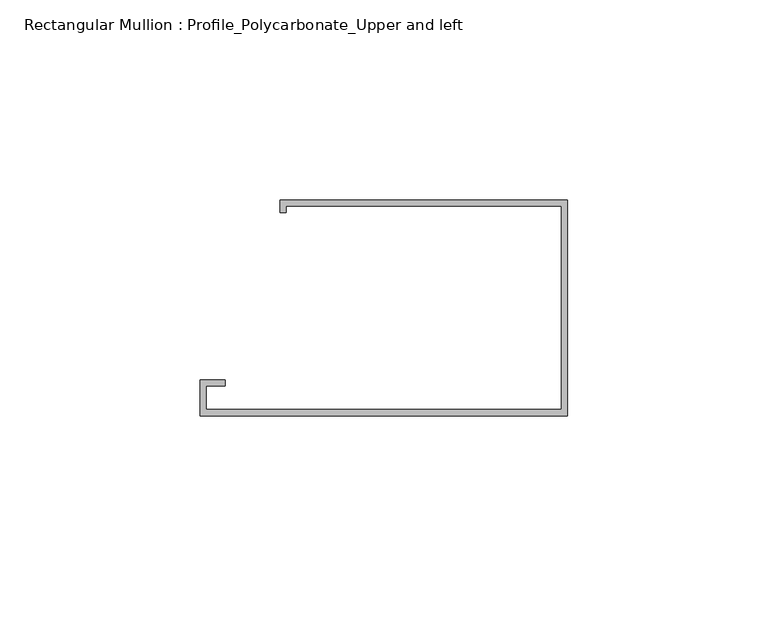
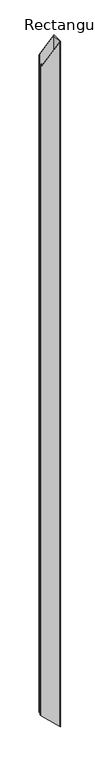
"""IFC4 building model written with IfcOpenShell, lengths in millimetres: member geometry, Rectangular Mullion : Profile_Polycarbonate_Upper and left."""

from ifc_helpers import new_model, si_unit, origin, place, context, project, spatial, faceted_brep, source, transform, mapped, element, save


def rectangular_mullion_profile_polycarbonate_upper_and_left_e2d1517f(model_context):
    return source(origin(), model_context, "Body", "Brep", [
        faceted_brep([(0.0, 25.015825, 0.0), (0.0, -28.984575, 0.0), (0.0, -28.984575, -3475.9884225), (0.0, 25.015825, -3475.9884225), (-71.9836, 25.015825, -75.0453753), (-71.9836, 25.015825, -3406.9416805), (-71.9836, 21.840825, -75.0453753), (-71.9836, 21.840825, -3406.9416805), (-70.3961, 21.840825, -73.3903521), (-70.3961, 21.840825, -3408.4644121), (-70.3961, 23.428325, -73.3903521), (-70.3961, 23.428325, -3408.4644121), (-1.5875, 23.428325, -1.6550233), (-1.5875, 23.428325, -3474.4656909), (-1.5875, -27.397075, -1.6550233), (-1.5875, -27.397075, -3474.4656909), (-90.4113, -27.397075, -94.2568855), (-90.4113, -27.397075, -3389.265812), (-90.4113, -21.580475, -94.2568855), (-90.4113, -21.580475, -3389.265812), (-85.6488, -21.580475, -89.2918157), (-85.6488, -21.580475, -3393.8340068), (-85.6488, -19.992975, -89.2918157), (-85.6488, -19.992975, -3393.8340068), (-91.9988, -19.992975, -95.9119088), (-91.9988, -19.992975, -3387.7430804), (-91.9988, -28.984575, -95.9119088), (-91.9988, -28.984575, -3387.7430804)], [[[0, 1, 2, 3]], [[4, 0, 3, 5]], [[6, 4, 5, 7]], [[8, 6, 7, 9]], [[10, 8, 9, 11]], [[12, 10, 11, 13]], [[14, 12, 13, 15]], [[16, 14, 15, 17]], [[18, 16, 17, 19]], [[20, 18, 19, 21]], [[22, 20, 21, 23]], [[24, 22, 23, 25]], [[26, 24, 25, 27]], [[1, 26, 27, 2]], [[1, 0, 4, 6, 8, 10, 12, 14, 16, 18, 20, 22, 24, 26]], [[2, 27, 25, 23, 21, 19, 17, 15, 13, 11, 9, 7, 5, 3]]]),
    ])


if __name__ == "__main__":
    model = new_model("IFC4")
    model_context = context("Model", 3, world=origin())
    ifc_project = project(units=[si_unit("LENGTHUNIT", "METRE", prefix="MILLI")], contexts=[model_context])
    site = spatial("IfcSite", under=ifc_project)
    building = spatial("IfcBuilding", under=site)
    placement = place(None, origin())
    rectangular_mullion_profile_polycarbonate_upper_and_left_shape = rectangular_mullion_profile_polycarbonate_upper_and_left_e2d1517f(model_context)
    element("IfcMember", 1, ObjectType="Rectangular Mullion : Profile_Polycarbonate_Upper and left", at=placement, inside=building, context=model_context, shape_type="MappedRepresentation", body=[
        mapped(rectangular_mullion_profile_polycarbonate_upper_and_left_shape, transform((0.0, 0.0, 0.0), x_axis=(1.0, 0.0, 0.0), y_axis=(0.0, 1.0, 0.0), z_axis=(0.0, 0.0, 1.0))),
    ])
    save(model, "model.ifc")

# Revit data of these elements
# Type "Rectangular Mullion : Profile_Polycarbonate_Upper and left"
#   built-in parameter 1007322 = 0.177167 (stored number, unit not read)
#   built-in parameter 1007321 = 0.00520833 (stored number, unit not read)
#   built-in parameter 1007320 = 0 (stored number, unit not read)
